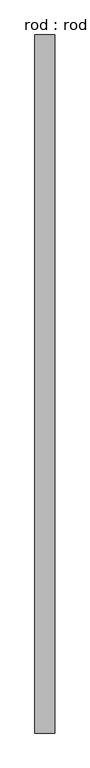
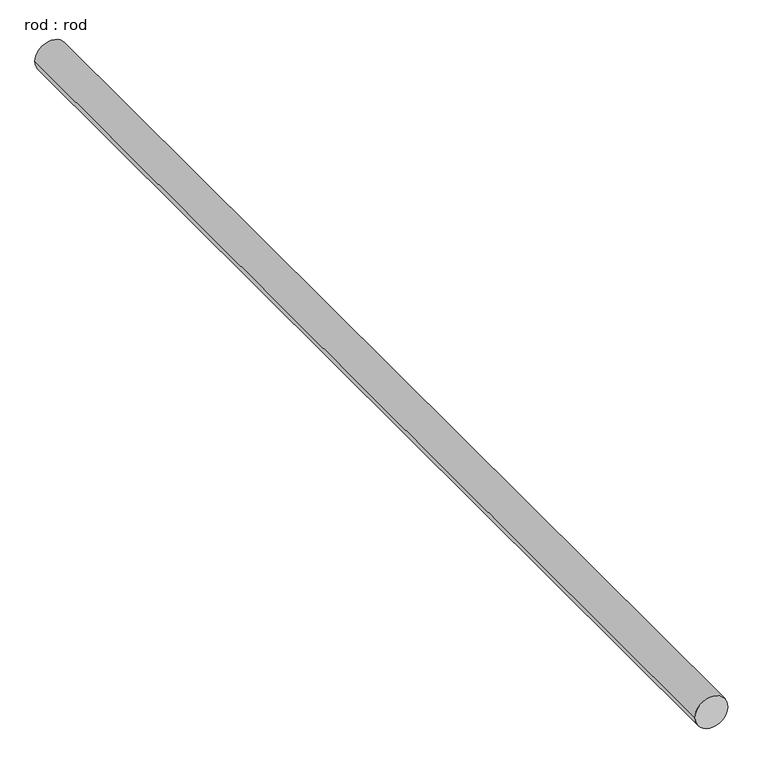
"""IFC4 building model written with IfcOpenShell, lengths in millimetres: proxy geometry, rod : rod."""

from ifc_helpers import new_model, si_unit, point, frame, frame_2d, origin, place, context, project, spatial, circle_curve, trimmed, segment, composite_curve, outline, extrude, source, transform, mapped, element, save


def rod_rod_2f2ad5b8(model_context):
    return source(origin(), model_context, "Body", "SweptSolid", [
        extrude(outline(composite_curve([segment(trimmed(circle_curve(frame_2d((0.0108462, 0.0)), 200.0), [point((0.0108462, 200.0))], [point((0.0108462, -200.0))], False, "CARTESIAN"), True, "CONTINUOUS"), segment(trimmed(circle_curve(frame_2d((0.0108462, 0.0)), 200.0), [point((0.0108462, -200.0))], [point((0.0108462, 200.0))], False, "CARTESIAN"), True, "CONTINUOUS")], self_intersect=False)), frame((0.0, -2871.5570989, 0.0), z_axis=(0.0, 1.0, 0.0), x_axis=(0.0, 0.0, 1.0)), (0.0, 0.0, 1.0), 13928.5714286),
    ])


if __name__ == "__main__":
    model = new_model("IFC4")
    model_context = context("Model", 3, world=origin())
    ifc_project = project(units=[si_unit("LENGTHUNIT", "METRE", prefix="MILLI")], contexts=[model_context])
    site = spatial("IfcSite", under=ifc_project)
    building = spatial("IfcBuilding", under=site)
    placement = place(None, origin())
    rod_rod_shape = rod_rod_2f2ad5b8(model_context)
    element("IfcBuildingElementProxy", 1, Name="rod : rod", ObjectType="rod : rod", at=placement, inside=building, context=model_context, shape_type="MappedRepresentation", body=[
        mapped(rod_rod_shape, transform((0.0, 0.0, 0.0), x_axis=(1.0, 0.0, 0.0), y_axis=(0.0, 1.0, 0.0), z_axis=(0.0, 0.0, 1.0))),
    ])
    save(model, "model.ifc")

# Revit data of these elements
# Type "rod : rod"
#   Default Elevation = 0
